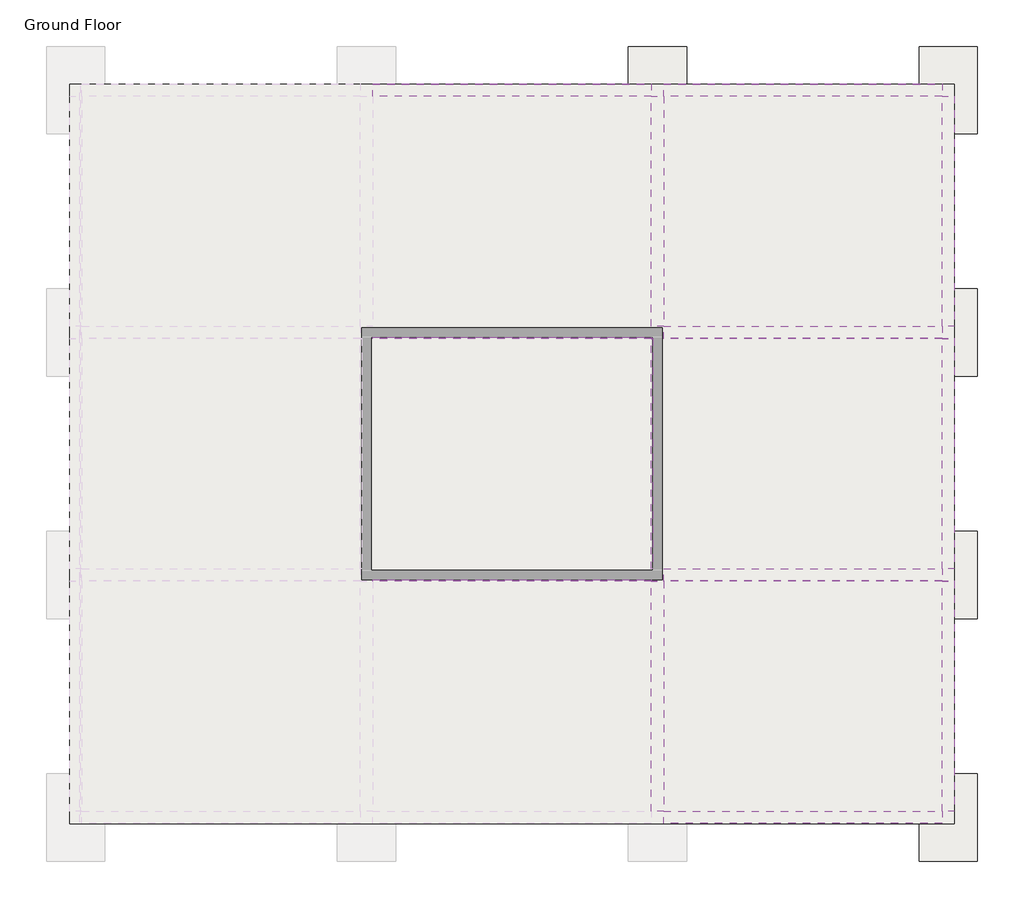
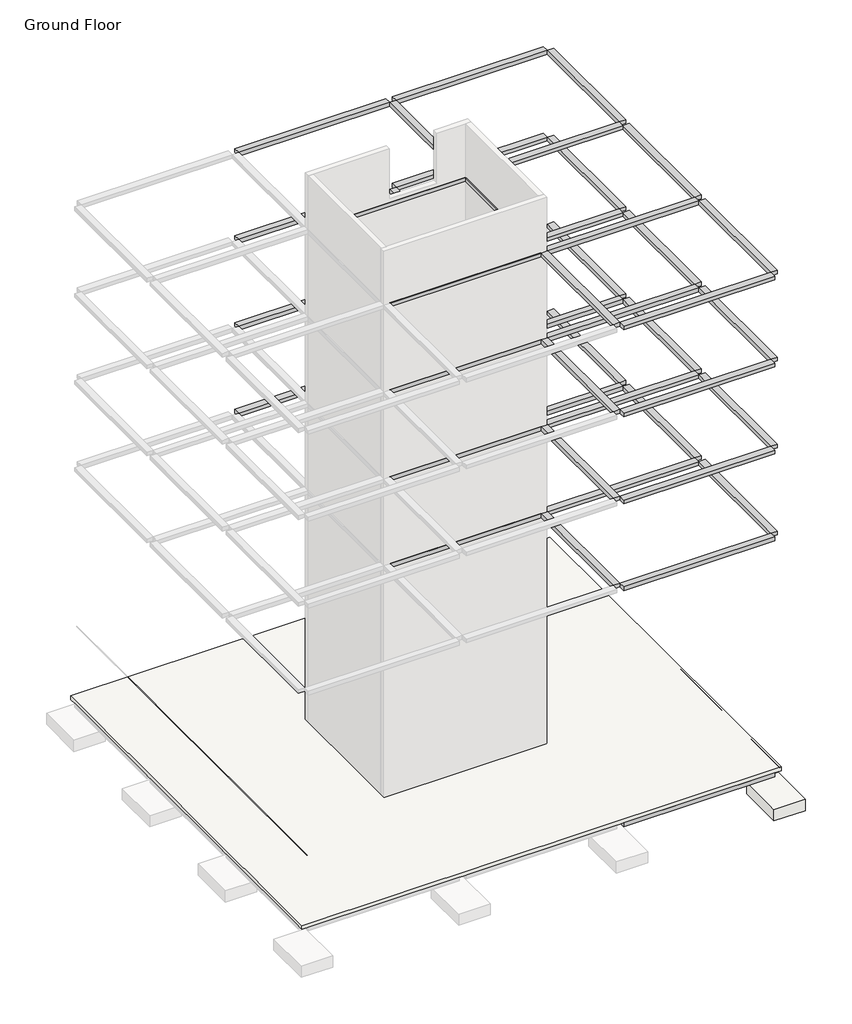
# One storey, part 2 of 3: 65 beams, 8 slabs.
"""IFC4 building model written with IfcOpenShell, lengths in millimetres."""

from ifc_helpers import new_model, si_unit, frame, origin, place, context, project, spatial, polyline, outline, extrude, faceted_brep, element, save

model = new_model("IFC4")

# Units and contexts
model_context = context("Model", 3, world=origin())
ifc_project = project(units=[si_unit("LENGTHUNIT", "METRE", prefix="MILLI")], contexts=[model_context])

# Site, building, storey
site = spatial("IfcSite", under=ifc_project)
building = spatial("IfcBuilding", under=site)
storey = spatial("IfcBuildingStorey", under=building, Name="Ground Floor", Elevation=2000.0)

# Beams
placement = place(None, origin())
element("IfcBeam", 1, ObjectType="Concrete-Rectangular Beam : 250 x 300mm", at=placement, inside=storey, context=model_context, shape_type="SweptSolid", body=[
    extrude(outline(polyline([(-2833.7181639, -5693.2383613), (-2833.7181639, -5443.2383613), (2916.2818361, -5443.2383613), (2916.2818361, -5693.2383613), (-2833.7181639, -5693.2383613)])), frame((0.0, 0.0, 1700.0), z_axis=(0.0, 0.0, 1.0), x_axis=(1.0, 0.0, 0.0)), (0.0, 0.0, 1.0), 150.0),
])
element("IfcBeam", 2, ObjectType="Concrete-Rectangular Beam : 250 x 300mm", at=placement, inside=storey, context=model_context, shape_type="SweptSolid", body=[
    extrude(outline(polyline([(3166.2818361, -5693.2383613), (3166.2818361, -5443.2383613), (8916.2818361, -5443.2383613), (8916.2818361, -5693.2383613), (3166.2818361, -5693.2383613)])), frame((0.0, 0.0, 1700.0), z_axis=(0.0, 0.0, 1.0), x_axis=(1.0, 0.0, 0.0)), (0.0, 0.0, 1.0), 150.0),
])
element("IfcBeam", 3, ObjectType="Concrete-Rectangular Beam : 250 x 300mm", at=placement, inside=storey, context=model_context, shape_type="SweptSolid", body=[
    extrude(outline(polyline([(3166.2818361, -10443.2383613), (2916.2818361, -10443.2383613), (2916.2818361, -5693.2383613), (3166.2818361, -5693.2383613), (3166.2818361, -10443.2383613)])), frame((0.0, 0.0, 1700.0), z_axis=(0.0, 0.0, 1.0), x_axis=(1.0, 0.0, 0.0)), (0.0, 0.0, 1.0), 150.0),
])
element("IfcBeam", 4, ObjectType="Concrete-Rectangular Beam : 250 x 300mm", at=placement, inside=storey, context=model_context, shape_type="SweptSolid", body=[
    extrude(outline(polyline([(2916.2818361, -15443.2383613), (2916.2818361, -10693.2383613), (2941.2818361, -10693.2383613), (2941.2818361, -15443.2383613), (2916.2818361, -15443.2383613)])), frame((0.0, 0.0, 1700.0), z_axis=(0.0, 0.0, 1.0), x_axis=(1.0, 0.0, 0.0)), (0.0, 0.0, 1.0), 150.0),
    extrude(outline(polyline([(3166.2818361, -10693.2383613), (3166.2818361, -15443.2383613), (3141.2818361, -15443.2383613), (3141.2818361, -10693.2383613), (3166.2818361, -10693.2383613)])), frame((0.0, 0.0, 1700.0), z_axis=(0.0, 0.0, 1.0), x_axis=(1.0, 0.0, 0.0)), (0.0, 0.0, 1.0), 150.0),
])
element("IfcBeam", 5, ObjectType="Concrete-Rectangular Beam : 250 x 300mm", at=placement, inside=storey, context=model_context, shape_type="SweptSolid", body=[
    extrude(outline(polyline([(3166.2818361, -20443.2383613), (2916.2818361, -20443.2383613), (2916.2818361, -15693.2383613), (3166.2818361, -15693.2383613), (3166.2818361, -20443.2383613)])), frame((0.0, 0.0, 1700.0), z_axis=(0.0, 0.0, 1.0), x_axis=(1.0, 0.0, 0.0)), (0.0, 0.0, 1.0), 150.0),
])
element("IfcBeam", 6, ObjectType="Concrete-Rectangular Beam : 250 x 300mm", at=placement, inside=storey, context=model_context, shape_type="SweptSolid", body=[
    extrude(outline(polyline([(9166.2818361, -10443.2383613), (8916.2818361, -10443.2383613), (8916.2818361, -5693.2383613), (9166.2818361, -5693.2383613), (9166.2818361, -10443.2383613)])), frame((0.0, 0.0, 1700.0), z_axis=(0.0, 0.0, 1.0), x_axis=(1.0, 0.0, 0.0)), (0.0, 0.0, 1.0), 150.0),
])
element("IfcBeam", 7, ObjectType="Concrete-Rectangular Beam : 250 x 300mm", at=placement, inside=storey, context=model_context, shape_type="SweptSolid", body=[
    extrude(outline(polyline([(9166.2818361, -15443.2383613), (8916.2818361, -15443.2383613), (8916.2818361, -10693.2383613), (9166.2818361, -10693.2383613), (9166.2818361, -15443.2383613)])), frame((0.0, 0.0, 1700.0), z_axis=(0.0, 0.0, 1.0), x_axis=(1.0, 0.0, 0.0)), (0.0, 0.0, 1.0), 150.0),
])
element("IfcBeam", 8, ObjectType="Concrete-Rectangular Beam : 250 x 300mm", at=placement, inside=storey, context=model_context, shape_type="SweptSolid", body=[
    extrude(outline(polyline([(9166.2818361, -20443.2383613), (8916.2818361, -20443.2383613), (8916.2818361, -15693.2383613), (9166.2818361, -15693.2383613), (9166.2818361, -20443.2383613)])), frame((0.0, 0.0, 1700.0), z_axis=(0.0, 0.0, 1.0), x_axis=(1.0, 0.0, 0.0)), (0.0, 0.0, 1.0), 150.0),
])
element("IfcBeam", 9, ObjectType="Concrete-Rectangular Beam : 250 x 300mm", at=placement, inside=storey, context=model_context, shape_type="SweptSolid", body=[
    extrude(outline(polyline([(3166.2818361, -20693.2383613), (3166.2818361, -20443.2383613), (8916.2818361, -20443.2383613), (8916.2818361, -20693.2383613), (3166.2818361, -20693.2383613)])), frame((0.0, 0.0, 1700.0), z_axis=(0.0, 0.0, 1.0), x_axis=(1.0, 0.0, 0.0)), (0.0, 0.0, 1.0), 150.0),
])
element("IfcBeam", 10, ObjectType="Concrete-Rectangular Beam : 250 x 300mm", at=placement, inside=storey, context=model_context, shape_type="SweptSolid", body=[
    extrude(outline(polyline([(2916.2818361, -15693.2383613), (-2833.7181639, -15693.2383613), (-2833.7181639, -15668.2383613), (2916.2818361, -15668.2383613), (2916.2818361, -15693.2383613)])), frame((0.0, 0.0, 1700.0), z_axis=(0.0, 0.0, 1.0), x_axis=(1.0, 0.0, 0.0)), (0.0, 0.0, 1.0), 150.0),
    extrude(outline(polyline([(-2833.7181639, -15443.2383613), (2916.2818361, -15443.2383613), (2916.2818361, -15468.2383613), (-2833.7181639, -15468.2383613), (-2833.7181639, -15443.2383613)])), frame((0.0, 0.0, 1700.0), z_axis=(0.0, 0.0, 1.0), x_axis=(1.0, 0.0, 0.0)), (0.0, 0.0, 1.0), 150.0),
])
element("IfcBeam", 11, ObjectType="Concrete-Rectangular Beam : 250 x 300mm", at=placement, inside=storey, context=model_context, shape_type="SweptSolid", body=[
    extrude(outline(polyline([(3166.2818361, -15693.2383613), (3166.2818361, -15443.2383613), (8916.2818361, -15443.2383613), (8916.2818361, -15693.2383613), (3166.2818361, -15693.2383613)])), frame((0.0, 0.0, 1700.0), z_axis=(0.0, 0.0, 1.0), x_axis=(1.0, 0.0, 0.0)), (0.0, 0.0, 1.0), 150.0),
])
element("IfcBeam", 12, ObjectType="Concrete-Rectangular Beam : 250 x 300mm", at=placement, inside=storey, context=model_context, shape_type="SweptSolid", body=[
    extrude(outline(polyline([(2916.2818361, -10693.2383613), (-2833.7181639, -10693.2383613), (-2833.7181639, -10668.2383613), (2916.2818361, -10668.2383613), (2916.2818361, -10693.2383613)])), frame((0.0, 0.0, 1700.0), z_axis=(0.0, 0.0, 1.0), x_axis=(1.0, 0.0, 0.0)), (0.0, 0.0, 1.0), 150.0),
    extrude(outline(polyline([(-2833.7181639, -10443.2383613), (2916.2818361, -10443.2383613), (2916.2818361, -10468.2383613), (-2833.7181639, -10468.2383613), (-2833.7181639, -10443.2383613)])), frame((0.0, 0.0, 1700.0), z_axis=(0.0, 0.0, 1.0), x_axis=(1.0, 0.0, 0.0)), (0.0, 0.0, 1.0), 150.0),
])
element("IfcBeam", 13, ObjectType="Concrete-Rectangular Beam : 250 x 300mm", at=placement, inside=storey, context=model_context, shape_type="SweptSolid", body=[
    extrude(outline(polyline([(3166.2818361, -10693.2383613), (3166.2818361, -10443.2383613), (8916.2818361, -10443.2383613), (8916.2818361, -10693.2383613), (3166.2818361, -10693.2383613)])), frame((0.0, 0.0, 1700.0), z_axis=(0.0, 0.0, 1.0), x_axis=(1.0, 0.0, 0.0)), (0.0, 0.0, 1.0), 150.0),
])
element("IfcBeam", 14, ObjectType="Concrete-Rectangular Beam : 250 x 300mm", at=placement, inside=storey, context=model_context, shape_type="SweptSolid", body=[
    extrude(outline(polyline([(-2833.7181639, -5693.2383613), (-2833.7181639, -5443.2383613), (2916.2818361, -5443.2383613), (2916.2818361, -5693.2383613), (-2833.7181639, -5693.2383613)])), frame((0.0, 0.0, 11200.0), z_axis=(0.0, 0.0, 1.0), x_axis=(1.0, 0.0, 0.0)), (0.0, 0.0, 1.0), 150.0),
])
element("IfcBeam", 15, ObjectType="Concrete-Rectangular Beam : 250 x 300mm", at=placement, inside=storey, context=model_context, shape_type="SweptSolid", body=[
    extrude(outline(polyline([(3166.2818361, -5693.2383613), (3166.2818361, -5443.2383613), (8916.2818361, -5443.2383613), (8916.2818361, -5693.2383613), (3166.2818361, -5693.2383613)])), frame((0.0, 0.0, 11200.0), z_axis=(0.0, 0.0, 1.0), x_axis=(1.0, 0.0, 0.0)), (0.0, 0.0, 1.0), 150.0),
])
element("IfcBeam", 16, ObjectType="Concrete-Rectangular Beam : 250 x 300mm", at=placement, inside=storey, context=model_context, shape_type="SweptSolid", body=[
    extrude(outline(polyline([(2916.2818361, -10443.2383613), (2916.2818361, -5693.2383613), (3166.2818361, -5693.2383613), (3166.2818361, -10443.2383613), (2916.2818361, -10443.2383613)])), frame((0.0, 0.0, 11200.0), z_axis=(0.0, 0.0, 1.0), x_axis=(1.0, 0.0, 0.0)), (0.0, 0.0, 1.0), 150.0),
])
element("IfcBeam", 17, ObjectType="Concrete-Rectangular Beam : 250 x 300mm", at=placement, inside=storey, context=model_context, shape_type="SweptSolid", body=[
    extrude(outline(polyline([(2916.2818361, -15443.2383613), (2916.2818361, -10693.2383613), (2941.2818361, -10693.2383613), (2941.2818361, -15443.2383613), (2916.2818361, -15443.2383613)])), frame((0.0, 0.0, 11200.0), z_axis=(0.0, 0.0, 1.0), x_axis=(1.0, 0.0, 0.0)), (0.0, 0.0, 1.0), 150.0),
    extrude(outline(polyline([(3166.2818361, -10693.2383613), (3166.2818361, -15443.2383613), (3141.2818361, -15443.2383613), (3141.2818361, -10693.2383613), (3166.2818361, -10693.2383613)])), frame((0.0, 0.0, 11200.0), z_axis=(0.0, 0.0, 1.0), x_axis=(1.0, 0.0, 0.0)), (0.0, 0.0, 1.0), 150.0),
])
element("IfcBeam", 18, ObjectType="Concrete-Rectangular Beam : 250 x 300mm", at=placement, inside=storey, context=model_context, shape_type="SweptSolid", body=[
    extrude(outline(polyline([(2916.2818361, -20443.2383613), (2916.2818361, -15693.2383613), (3166.2818361, -15693.2383613), (3166.2818361, -20443.2383613), (2916.2818361, -20443.2383613)])), frame((0.0, 0.0, 11200.0), z_axis=(0.0, 0.0, 1.0), x_axis=(1.0, 0.0, 0.0)), (0.0, 0.0, 1.0), 150.0),
])
element("IfcBeam", 19, ObjectType="Concrete-Rectangular Beam : 250 x 300mm", at=placement, inside=storey, context=model_context, shape_type="SweptSolid", body=[
    extrude(outline(polyline([(8916.2818361, -10443.2383613), (8916.2818361, -5693.2383613), (9166.2818361, -5693.2383613), (9166.2818361, -10443.2383613), (8916.2818361, -10443.2383613)])), frame((0.0, 0.0, 11200.0), z_axis=(0.0, 0.0, 1.0), x_axis=(1.0, 0.0, 0.0)), (0.0, 0.0, 1.0), 150.0),
])
element("IfcBeam", 20, ObjectType="Concrete-Rectangular Beam : 250 x 300mm", at=placement, inside=storey, context=model_context, shape_type="SweptSolid", body=[
    extrude(outline(polyline([(8916.2818361, -15443.2383613), (8916.2818361, -10693.2383613), (9166.2818361, -10693.2383613), (9166.2818361, -15443.2383613), (8916.2818361, -15443.2383613)])), frame((0.0, 0.0, 11200.0), z_axis=(0.0, 0.0, 1.0), x_axis=(1.0, 0.0, 0.0)), (0.0, 0.0, 1.0), 150.0),
])
element("IfcBeam", 21, ObjectType="Concrete-Rectangular Beam : 250 x 300mm", at=placement, inside=storey, context=model_context, shape_type="SweptSolid", body=[
    extrude(outline(polyline([(8916.2818361, -20443.2383613), (8916.2818361, -15693.2383613), (9166.2818361, -15693.2383613), (9166.2818361, -20443.2383613), (8916.2818361, -20443.2383613)])), frame((0.0, 0.0, 11200.0), z_axis=(0.0, 0.0, 1.0), x_axis=(1.0, 0.0, 0.0)), (0.0, 0.0, 1.0), 150.0),
])
element("IfcBeam", 22, ObjectType="Concrete-Rectangular Beam : 250 x 300mm", at=placement, inside=storey, context=model_context, shape_type="SweptSolid", body=[
    extrude(outline(polyline([(3166.2818361, -20443.2383613), (8916.2818361, -20443.2383613), (8916.2818361, -20693.2383613), (3166.2818361, -20693.2383613), (3166.2818361, -20443.2383613)])), frame((0.0, 0.0, 11200.0), z_axis=(0.0, 0.0, 1.0), x_axis=(1.0, 0.0, 0.0)), (0.0, 0.0, 1.0), 150.0),
])
element("IfcBeam", 23, ObjectType="Concrete-Rectangular Beam : 250 x 300mm", at=placement, inside=storey, context=model_context, shape_type="SweptSolid", body=[
    extrude(outline(polyline([(2916.2818361, -15693.2383613), (-2833.7181639, -15693.2383613), (-2833.7181639, -15668.2383613), (2916.2818361, -15668.2383613), (2916.2818361, -15693.2383613)])), frame((0.0, 0.0, 11200.0), z_axis=(0.0, 0.0, 1.0), x_axis=(1.0, 0.0, 0.0)), (0.0, 0.0, 1.0), 150.0),
    extrude(outline(polyline([(-2833.7181639, -15443.2383613), (2916.2818361, -15443.2383613), (2916.2818361, -15468.2383613), (-2833.7181639, -15468.2383613), (-2833.7181639, -15443.2383613)])), frame((0.0, 0.0, 11200.0), z_axis=(0.0, 0.0, 1.0), x_axis=(1.0, 0.0, 0.0)), (0.0, 0.0, 1.0), 150.0),
])
element("IfcBeam", 24, ObjectType="Concrete-Rectangular Beam : 250 x 300mm", at=placement, inside=storey, context=model_context, shape_type="SweptSolid", body=[
    extrude(outline(polyline([(3166.2818361, -15693.2383613), (3166.2818361, -15443.2383613), (8916.2818361, -15443.2383613), (8916.2818361, -15693.2383613), (3166.2818361, -15693.2383613)])), frame((0.0, 0.0, 11200.0), z_axis=(0.0, 0.0, 1.0), x_axis=(1.0, 0.0, 0.0)), (0.0, 0.0, 1.0), 150.0),
])
element("IfcBeam", 25, ObjectType="Concrete-Rectangular Beam : 250 x 300mm", at=placement, inside=storey, context=model_context, shape_type="SweptSolid", body=[
    extrude(outline(polyline([(2916.2818361, -10693.2383613), (-2833.7181639, -10693.2383613), (-2833.7181639, -10668.2383613), (2916.2818361, -10668.2383613), (2916.2818361, -10693.2383613)])), frame((0.0, 0.0, 11200.0), z_axis=(0.0, 0.0, 1.0), x_axis=(1.0, 0.0, 0.0)), (0.0, 0.0, 1.0), 150.0),
    extrude(outline(polyline([(-2833.7181639, -10443.2383613), (2916.2818361, -10443.2383613), (2916.2818361, -10468.2383613), (-2833.7181639, -10468.2383613), (-2833.7181639, -10443.2383613)])), frame((0.0, 0.0, 11200.0), z_axis=(0.0, 0.0, 1.0), x_axis=(1.0, 0.0, 0.0)), (0.0, 0.0, 1.0), 150.0),
])
element("IfcBeam", 26, ObjectType="Concrete-Rectangular Beam : 250 x 300mm", at=placement, inside=storey, context=model_context, shape_type="SweptSolid", body=[
    extrude(outline(polyline([(3166.2818361, -10693.2383613), (3166.2818361, -10443.2383613), (8916.2818361, -10443.2383613), (8916.2818361, -10693.2383613), (3166.2818361, -10693.2383613)])), frame((0.0, 0.0, 11200.0), z_axis=(0.0, 0.0, 1.0), x_axis=(1.0, 0.0, 0.0)), (0.0, 0.0, 1.0), 150.0),
])
element("IfcBeam", 27, ObjectType="Concrete-Rectangular Beam : 250 x 300mm", at=placement, inside=storey, context=model_context, shape_type="SweptSolid", body=[
    extrude(outline(polyline([(-2833.7181639, -5693.2383613), (-2833.7181639, -5443.2383613), (2916.2818361, -5443.2383613), (2916.2818361, -5693.2383613), (-2833.7181639, -5693.2383613)])), frame((0.0, 0.0, 14700.0), z_axis=(0.0, 0.0, 1.0), x_axis=(1.0, 0.0, 0.0)), (0.0, 0.0, 1.0), 150.0),
])
element("IfcBeam", 28, ObjectType="Concrete-Rectangular Beam : 250 x 300mm", at=placement, inside=storey, context=model_context, shape_type="SweptSolid", body=[
    extrude(outline(polyline([(3166.2818361, -5693.2383613), (3166.2818361, -5443.2383613), (8916.2818361, -5443.2383613), (8916.2818361, -5693.2383613), (3166.2818361, -5693.2383613)])), frame((0.0, 0.0, 14700.0), z_axis=(0.0, 0.0, 1.0), x_axis=(1.0, 0.0, 0.0)), (0.0, 0.0, 1.0), 150.0),
])
element("IfcBeam", 29, ObjectType="Concrete-Rectangular Beam : 250 x 300mm", at=placement, inside=storey, context=model_context, shape_type="SweptSolid", body=[
    extrude(outline(polyline([(2916.2818361, -10443.2383613), (2916.2818361, -5693.2383613), (3166.2818361, -5693.2383613), (3166.2818361, -10443.2383613), (2916.2818361, -10443.2383613)])), frame((0.0, 0.0, 14700.0), z_axis=(0.0, 0.0, 1.0), x_axis=(1.0, 0.0, 0.0)), (0.0, 0.0, 1.0), 150.0),
])
element("IfcBeam", 30, ObjectType="Concrete-Rectangular Beam : 250 x 300mm", at=placement, inside=storey, context=model_context, shape_type="SweptSolid", body=[
    extrude(outline(polyline([(2916.2818361, -15443.2383613), (2916.2818361, -10693.2383613), (2941.2818361, -10693.2383613), (2941.2818361, -15443.2383613), (2916.2818361, -15443.2383613)])), frame((0.0, 0.0, 14700.0), z_axis=(0.0, 0.0, 1.0), x_axis=(1.0, 0.0, 0.0)), (0.0, 0.0, 1.0), 150.0),
    extrude(outline(polyline([(3166.2818361, -10693.2383613), (3166.2818361, -15443.2383613), (3141.2818361, -15443.2383613), (3141.2818361, -10693.2383613), (3166.2818361, -10693.2383613)])), frame((0.0, 0.0, 14700.0), z_axis=(0.0, 0.0, 1.0), x_axis=(1.0, 0.0, 0.0)), (0.0, 0.0, 1.0), 150.0),
])
element("IfcBeam", 31, ObjectType="Concrete-Rectangular Beam : 250 x 300mm", at=placement, inside=storey, context=model_context, shape_type="SweptSolid", body=[
    extrude(outline(polyline([(2916.2818361, -20443.2383613), (2916.2818361, -15693.2383613), (3166.2818361, -15693.2383613), (3166.2818361, -20443.2383613), (2916.2818361, -20443.2383613)])), frame((0.0, 0.0, 14700.0), z_axis=(0.0, 0.0, 1.0), x_axis=(1.0, 0.0, 0.0)), (0.0, 0.0, 1.0), 150.0),
])
element("IfcBeam", 32, ObjectType="Concrete-Rectangular Beam : 250 x 300mm", at=placement, inside=storey, context=model_context, shape_type="SweptSolid", body=[
    extrude(outline(polyline([(8916.2818361, -10443.2383613), (8916.2818361, -5693.2383613), (9166.2818361, -5693.2383613), (9166.2818361, -10443.2383613), (8916.2818361, -10443.2383613)])), frame((0.0, 0.0, 14700.0), z_axis=(0.0, 0.0, 1.0), x_axis=(1.0, 0.0, 0.0)), (0.0, 0.0, 1.0), 150.0),
])
element("IfcBeam", 33, ObjectType="Concrete-Rectangular Beam : 250 x 300mm", at=placement, inside=storey, context=model_context, shape_type="SweptSolid", body=[
    extrude(outline(polyline([(8916.2818361, -15443.2383613), (8916.2818361, -10693.2383613), (9166.2818361, -10693.2383613), (9166.2818361, -15443.2383613), (8916.2818361, -15443.2383613)])), frame((0.0, 0.0, 14700.0), z_axis=(0.0, 0.0, 1.0), x_axis=(1.0, 0.0, 0.0)), (0.0, 0.0, 1.0), 150.0),
])
element("IfcBeam", 34, ObjectType="Concrete-Rectangular Beam : 250 x 300mm", at=placement, inside=storey, context=model_context, shape_type="SweptSolid", body=[
    extrude(outline(polyline([(8916.2818361, -20443.2383613), (8916.2818361, -15693.2383613), (9166.2818361, -15693.2383613), (9166.2818361, -20443.2383613), (8916.2818361, -20443.2383613)])), frame((0.0, 0.0, 14700.0), z_axis=(0.0, 0.0, 1.0), x_axis=(1.0, 0.0, 0.0)), (0.0, 0.0, 1.0), 150.0),
])
element("IfcBeam", 35, ObjectType="Concrete-Rectangular Beam : 250 x 300mm", at=placement, inside=storey, context=model_context, shape_type="SweptSolid", body=[
    extrude(outline(polyline([(3166.2818361, -20443.2383613), (8916.2818361, -20443.2383613), (8916.2818361, -20693.2383613), (3166.2818361, -20693.2383613), (3166.2818361, -20443.2383613)])), frame((0.0, 0.0, 14700.0), z_axis=(0.0, 0.0, 1.0), x_axis=(1.0, 0.0, 0.0)), (0.0, 0.0, 1.0), 150.0),
])
element("IfcBeam", 36, ObjectType="Concrete-Rectangular Beam : 250 x 300mm", at=placement, inside=storey, context=model_context, shape_type="SweptSolid", body=[
    extrude(outline(polyline([(2916.2818361, -15693.2383613), (-2833.7181639, -15693.2383613), (-2833.7181639, -15668.2383613), (2916.2818361, -15668.2383613), (2916.2818361, -15693.2383613)])), frame((0.0, 0.0, 14700.0), z_axis=(0.0, 0.0, 1.0), x_axis=(1.0, 0.0, 0.0)), (0.0, 0.0, 1.0), 150.0),
    extrude(outline(polyline([(-2833.7181639, -15443.2383613), (2916.2818361, -15443.2383613), (2916.2818361, -15468.2383613), (-2833.7181639, -15468.2383613), (-2833.7181639, -15443.2383613)])), frame((0.0, 0.0, 14700.0), z_axis=(0.0, 0.0, 1.0), x_axis=(1.0, 0.0, 0.0)), (0.0, 0.0, 1.0), 150.0),
])
element("IfcBeam", 37, ObjectType="Concrete-Rectangular Beam : 250 x 300mm", at=placement, inside=storey, context=model_context, shape_type="SweptSolid", body=[
    extrude(outline(polyline([(3166.2818361, -15693.2383613), (3166.2818361, -15443.2383613), (8916.2818361, -15443.2383613), (8916.2818361, -15693.2383613), (3166.2818361, -15693.2383613)])), frame((0.0, 0.0, 14700.0), z_axis=(0.0, 0.0, 1.0), x_axis=(1.0, 0.0, 0.0)), (0.0, 0.0, 1.0), 150.0),
])
element("IfcBeam", 38, ObjectType="Concrete-Rectangular Beam : 250 x 300mm", at=placement, inside=storey, context=model_context, shape_type="SweptSolid", body=[
    extrude(outline(polyline([(2916.2818361, -10693.2383613), (-2833.7181639, -10693.2383613), (-2833.7181639, -10668.2383613), (2916.2818361, -10668.2383613), (2916.2818361, -10693.2383613)])), frame((0.0, 0.0, 14700.0), z_axis=(0.0, 0.0, 1.0), x_axis=(1.0, 0.0, 0.0)), (0.0, 0.0, 1.0), 150.0),
    extrude(outline(polyline([(-2833.7181639, -10443.2383613), (2916.2818361, -10443.2383613), (2916.2818361, -10468.2383613), (-2833.7181639, -10468.2383613), (-2833.7181639, -10443.2383613)])), frame((0.0, 0.0, 14700.0), z_axis=(0.0, 0.0, 1.0), x_axis=(1.0, 0.0, 0.0)), (0.0, 0.0, 1.0), 150.0),
])
element("IfcBeam", 39, ObjectType="Concrete-Rectangular Beam : 250 x 300mm", at=placement, inside=storey, context=model_context, shape_type="SweptSolid", body=[
    extrude(outline(polyline([(3166.2818361, -10693.2383613), (3166.2818361, -10443.2383613), (8916.2818361, -10443.2383613), (8916.2818361, -10693.2383613), (3166.2818361, -10693.2383613)])), frame((0.0, 0.0, 14700.0), z_axis=(0.0, 0.0, 1.0), x_axis=(1.0, 0.0, 0.0)), (0.0, 0.0, 1.0), 150.0),
])
element("IfcBeam", 40, ObjectType="Concrete-Rectangular Beam : 250 x 300mm", at=placement, inside=storey, context=model_context, shape_type="SweptSolid", body=[
    extrude(outline(polyline([(-2833.7181639, -5693.2383613), (-2833.7181639, -5443.2383613), (2916.2818361, -5443.2383613), (2916.2818361, -5693.2383613), (-2833.7181639, -5693.2383613)])), frame((0.0, 0.0, 18200.0), z_axis=(0.0, 0.0, 1.0), x_axis=(1.0, 0.0, 0.0)), (0.0, 0.0, 1.0), 150.0),
])
element("IfcBeam", 41, ObjectType="Concrete-Rectangular Beam : 250 x 300mm", at=placement, inside=storey, context=model_context, shape_type="SweptSolid", body=[
    extrude(outline(polyline([(3166.2818361, -5693.2383613), (3166.2818361, -5443.2383613), (8916.2818361, -5443.2383613), (8916.2818361, -5693.2383613), (3166.2818361, -5693.2383613)])), frame((0.0, 0.0, 18200.0), z_axis=(0.0, 0.0, 1.0), x_axis=(1.0, 0.0, 0.0)), (0.0, 0.0, 1.0), 150.0),
])
element("IfcBeam", 42, ObjectType="Concrete-Rectangular Beam : 250 x 300mm", at=placement, inside=storey, context=model_context, shape_type="SweptSolid", body=[
    extrude(outline(polyline([(2916.2818361, -10443.2383613), (2916.2818361, -5693.2383613), (3166.2818361, -5693.2383613), (3166.2818361, -10443.2383613), (2916.2818361, -10443.2383613)])), frame((0.0, 0.0, 18200.0), z_axis=(0.0, 0.0, 1.0), x_axis=(1.0, 0.0, 0.0)), (0.0, 0.0, 1.0), 150.0),
])
element("IfcBeam", 43, ObjectType="Concrete-Rectangular Beam : 250 x 300mm", at=placement, inside=storey, context=model_context, shape_type="SweptSolid", body=[
    extrude(outline(polyline([(2916.2818361, -15443.2383613), (2916.2818361, -10693.2383613), (2941.2818361, -10693.2383613), (2941.2818361, -15443.2383613), (2916.2818361, -15443.2383613)])), frame((0.0, 0.0, 18200.0), z_axis=(0.0, 0.0, 1.0), x_axis=(1.0, 0.0, 0.0)), (0.0, 0.0, 1.0), 150.0),
    extrude(outline(polyline([(3166.2818361, -10693.2383613), (3166.2818361, -15443.2383613), (3141.2818361, -15443.2383613), (3141.2818361, -10693.2383613), (3166.2818361, -10693.2383613)])), frame((0.0, 0.0, 18200.0), z_axis=(0.0, 0.0, 1.0), x_axis=(1.0, 0.0, 0.0)), (0.0, 0.0, 1.0), 150.0),
])
element("IfcBeam", 44, ObjectType="Concrete-Rectangular Beam : 250 x 300mm", at=placement, inside=storey, context=model_context, shape_type="SweptSolid", body=[
    extrude(outline(polyline([(2916.2818361, -20443.2383613), (2916.2818361, -15693.2383613), (3166.2818361, -15693.2383613), (3166.2818361, -20443.2383613), (2916.2818361, -20443.2383613)])), frame((0.0, 0.0, 18200.0), z_axis=(0.0, 0.0, 1.0), x_axis=(1.0, 0.0, 0.0)), (0.0, 0.0, 1.0), 150.0),
])
element("IfcBeam", 45, ObjectType="Concrete-Rectangular Beam : 250 x 300mm", at=placement, inside=storey, context=model_context, shape_type="SweptSolid", body=[
    extrude(outline(polyline([(8916.2818361, -10443.2383613), (8916.2818361, -5693.2383613), (9166.2818361, -5693.2383613), (9166.2818361, -10443.2383613), (8916.2818361, -10443.2383613)])), frame((0.0, 0.0, 18200.0), z_axis=(0.0, 0.0, 1.0), x_axis=(1.0, 0.0, 0.0)), (0.0, 0.0, 1.0), 150.0),
])
element("IfcBeam", 46, ObjectType="Concrete-Rectangular Beam : 250 x 300mm", at=placement, inside=storey, context=model_context, shape_type="SweptSolid", body=[
    extrude(outline(polyline([(8916.2818361, -15443.2383613), (8916.2818361, -10693.2383613), (9166.2818361, -10693.2383613), (9166.2818361, -15443.2383613), (8916.2818361, -15443.2383613)])), frame((0.0, 0.0, 18200.0), z_axis=(0.0, 0.0, 1.0), x_axis=(1.0, 0.0, 0.0)), (0.0, 0.0, 1.0), 150.0),
])
element("IfcBeam", 47, ObjectType="Concrete-Rectangular Beam : 250 x 300mm", at=placement, inside=storey, context=model_context, shape_type="SweptSolid", body=[
    extrude(outline(polyline([(8916.2818361, -20443.2383613), (8916.2818361, -15693.2383613), (9166.2818361, -15693.2383613), (9166.2818361, -20443.2383613), (8916.2818361, -20443.2383613)])), frame((0.0, 0.0, 18200.0), z_axis=(0.0, 0.0, 1.0), x_axis=(1.0, 0.0, 0.0)), (0.0, 0.0, 1.0), 150.0),
])
element("IfcBeam", 48, ObjectType="Concrete-Rectangular Beam : 250 x 300mm", at=placement, inside=storey, context=model_context, shape_type="SweptSolid", body=[
    extrude(outline(polyline([(3166.2818361, -20443.2383613), (8916.2818361, -20443.2383613), (8916.2818361, -20693.2383613), (3166.2818361, -20693.2383613), (3166.2818361, -20443.2383613)])), frame((0.0, 0.0, 18200.0), z_axis=(0.0, 0.0, 1.0), x_axis=(1.0, 0.0, 0.0)), (0.0, 0.0, 1.0), 150.0),
])
element("IfcBeam", 49, ObjectType="Concrete-Rectangular Beam : 250 x 300mm", at=placement, inside=storey, context=model_context, shape_type="SweptSolid", body=[
    extrude(outline(polyline([(2916.2818361, -15693.2383613), (-2833.7181639, -15693.2383613), (-2833.7181639, -15668.2383613), (2916.2818361, -15668.2383613), (2916.2818361, -15693.2383613)])), frame((0.0, 0.0, 18200.0), z_axis=(0.0, 0.0, 1.0), x_axis=(1.0, 0.0, 0.0)), (0.0, 0.0, 1.0), 150.0),
    extrude(outline(polyline([(-2833.7181639, -15443.2383613), (2916.2818361, -15443.2383613), (2916.2818361, -15468.2383613), (-2833.7181639, -15468.2383613), (-2833.7181639, -15443.2383613)])), frame((0.0, 0.0, 18200.0), z_axis=(0.0, 0.0, 1.0), x_axis=(1.0, 0.0, 0.0)), (0.0, 0.0, 1.0), 150.0),
])
element("IfcBeam", 50, ObjectType="Concrete-Rectangular Beam : 250 x 300mm", at=placement, inside=storey, context=model_context, shape_type="SweptSolid", body=[
    extrude(outline(polyline([(3166.2818361, -15693.2383613), (3166.2818361, -15443.2383613), (8916.2818361, -15443.2383613), (8916.2818361, -15693.2383613), (3166.2818361, -15693.2383613)])), frame((0.0, 0.0, 18200.0), z_axis=(0.0, 0.0, 1.0), x_axis=(1.0, 0.0, 0.0)), (0.0, 0.0, 1.0), 150.0),
])
element("IfcBeam", 51, ObjectType="Concrete-Rectangular Beam : 250 x 300mm", at=placement, inside=storey, context=model_context, shape_type="SweptSolid", body=[
    extrude(outline(polyline([(2916.2818361, -10693.2383613), (-2833.7181639, -10693.2383613), (-2833.7181639, -10668.2383613), (2916.2818361, -10668.2383613), (2916.2818361, -10693.2383613)])), frame((0.0, 0.0, 18200.0), z_axis=(0.0, 0.0, 1.0), x_axis=(1.0, 0.0, 0.0)), (0.0, 0.0, 1.0), 150.0),
    extrude(outline(polyline([(-2833.7181639, -10443.2383613), (2916.2818361, -10443.2383613), (2916.2818361, -10468.2383613), (-2833.7181639, -10468.2383613), (-2833.7181639, -10443.2383613)])), frame((0.0, 0.0, 18200.0), z_axis=(0.0, 0.0, 1.0), x_axis=(1.0, 0.0, 0.0)), (0.0, 0.0, 1.0), 150.0),
])
element("IfcBeam", 52, ObjectType="Concrete-Rectangular Beam : 250 x 300mm", at=placement, inside=storey, context=model_context, shape_type="SweptSolid", body=[
    extrude(outline(polyline([(3166.2818361, -10693.2383613), (3166.2818361, -10443.2383613), (8916.2818361, -10443.2383613), (8916.2818361, -10693.2383613), (3166.2818361, -10693.2383613)])), frame((0.0, 0.0, 18200.0), z_axis=(0.0, 0.0, 1.0), x_axis=(1.0, 0.0, 0.0)), (0.0, 0.0, 1.0), 150.0),
])
element("IfcBeam", 53, ObjectType="Concrete-Rectangular Beam : 250 x 300mm", at=placement, inside=storey, context=model_context, shape_type="SweptSolid", body=[
    extrude(outline(polyline([(-2833.7181639, -5693.2383613), (-2833.7181639, -5443.2383613), (2916.2818361, -5443.2383613), (2916.2818361, -5693.2383613), (-2833.7181639, -5693.2383613)])), frame((0.0, 0.0, 21700.0), z_axis=(0.0, 0.0, 1.0), x_axis=(1.0, 0.0, 0.0)), (0.0, 0.0, 1.0), 150.0),
])
element("IfcBeam", 54, ObjectType="Concrete-Rectangular Beam : 250 x 300mm", at=placement, inside=storey, context=model_context, shape_type="SweptSolid", body=[
    extrude(outline(polyline([(3166.2818361, -5693.2383613), (3166.2818361, -5443.2383613), (8916.2818361, -5443.2383613), (8916.2818361, -5693.2383613), (3166.2818361, -5693.2383613)])), frame((0.0, 0.0, 21700.0), z_axis=(0.0, 0.0, 1.0), x_axis=(1.0, 0.0, 0.0)), (0.0, 0.0, 1.0), 150.0),
])
element("IfcBeam", 55, ObjectType="Concrete-Rectangular Beam : 250 x 300mm", at=placement, inside=storey, context=model_context, shape_type="SweptSolid", body=[
    extrude(outline(polyline([(2916.2818361, -10443.2383613), (2916.2818361, -5693.2383613), (3166.2818361, -5693.2383613), (3166.2818361, -10443.2383613), (2916.2818361, -10443.2383613)])), frame((0.0, 0.0, 21700.0), z_axis=(0.0, 0.0, 1.0), x_axis=(1.0, 0.0, 0.0)), (0.0, 0.0, 1.0), 150.0),
])
element("IfcBeam", 56, ObjectType="Concrete-Rectangular Beam : 250 x 300mm", at=placement, inside=storey, context=model_context, shape_type="SweptSolid", body=[
    extrude(outline(polyline([(2916.2818361, -15443.2383613), (2916.2818361, -10693.2383613), (2941.2818361, -10693.2383613), (2941.2818361, -15443.2383613), (2916.2818361, -15443.2383613)])), frame((0.0, 0.0, 21700.0), z_axis=(0.0, 0.0, 1.0), x_axis=(1.0, 0.0, 0.0)), (0.0, 0.0, 1.0), 150.0),
    extrude(outline(polyline([(3166.2818361, -10693.2383613), (3166.2818361, -15443.2383613), (3141.2818361, -15443.2383613), (3141.2818361, -10693.2383613), (3166.2818361, -10693.2383613)])), frame((0.0, 0.0, 21700.0), z_axis=(0.0, 0.0, 1.0), x_axis=(1.0, 0.0, 0.0)), (0.0, 0.0, 1.0), 150.0),
])
element("IfcBeam", 57, ObjectType="Concrete-Rectangular Beam : 250 x 300mm", at=placement, inside=storey, context=model_context, shape_type="SweptSolid", body=[
    extrude(outline(polyline([(2916.2818361, -20443.2383613), (2916.2818361, -15693.2383613), (3166.2818361, -15693.2383613), (3166.2818361, -20443.2383613), (2916.2818361, -20443.2383613)])), frame((0.0, 0.0, 21700.0), z_axis=(0.0, 0.0, 1.0), x_axis=(1.0, 0.0, 0.0)), (0.0, 0.0, 1.0), 150.0),
])
element("IfcBeam", 58, ObjectType="Concrete-Rectangular Beam : 250 x 300mm", at=placement, inside=storey, context=model_context, shape_type="SweptSolid", body=[
    extrude(outline(polyline([(8916.2818361, -10443.2383613), (8916.2818361, -5693.2383613), (9166.2818361, -5693.2383613), (9166.2818361, -10443.2383613), (8916.2818361, -10443.2383613)])), frame((0.0, 0.0, 21700.0), z_axis=(0.0, 0.0, 1.0), x_axis=(1.0, 0.0, 0.0)), (0.0, 0.0, 1.0), 150.0),
])
element("IfcBeam", 59, ObjectType="Concrete-Rectangular Beam : 250 x 300mm", at=placement, inside=storey, context=model_context, shape_type="SweptSolid", body=[
    extrude(outline(polyline([(8916.2818361, -15443.2383613), (8916.2818361, -10693.2383613), (9166.2818361, -10693.2383613), (9166.2818361, -15443.2383613), (8916.2818361, -15443.2383613)])), frame((0.0, 0.0, 21700.0), z_axis=(0.0, 0.0, 1.0), x_axis=(1.0, 0.0, 0.0)), (0.0, 0.0, 1.0), 150.0),
])
element("IfcBeam", 60, ObjectType="Concrete-Rectangular Beam : 250 x 300mm", at=placement, inside=storey, context=model_context, shape_type="SweptSolid", body=[
    extrude(outline(polyline([(8916.2818361, -20443.2383613), (8916.2818361, -15693.2383613), (9166.2818361, -15693.2383613), (9166.2818361, -20443.2383613), (8916.2818361, -20443.2383613)])), frame((0.0, 0.0, 21700.0), z_axis=(0.0, 0.0, 1.0), x_axis=(1.0, 0.0, 0.0)), (0.0, 0.0, 1.0), 150.0),
])
element("IfcBeam", 61, ObjectType="Concrete-Rectangular Beam : 250 x 300mm", at=placement, inside=storey, context=model_context, shape_type="SweptSolid", body=[
    extrude(outline(polyline([(3166.2818361, -20443.2383613), (8916.2818361, -20443.2383613), (8916.2818361, -20693.2383613), (3166.2818361, -20693.2383613), (3166.2818361, -20443.2383613)])), frame((0.0, 0.0, 21700.0), z_axis=(0.0, 0.0, 1.0), x_axis=(1.0, 0.0, 0.0)), (0.0, 0.0, 1.0), 150.0),
])
element("IfcBeam", 62, ObjectType="Concrete-Rectangular Beam : 250 x 300mm", at=placement, inside=storey, context=model_context, shape_type="SweptSolid", body=[
    extrude(outline(polyline([(2916.2818361, -15693.2383613), (-2833.7181639, -15693.2383613), (-2833.7181639, -15668.2383613), (2916.2818361, -15668.2383613), (2916.2818361, -15693.2383613)])), frame((0.0, 0.0, 21700.0), z_axis=(0.0, 0.0, 1.0), x_axis=(1.0, 0.0, 0.0)), (0.0, 0.0, 1.0), 150.0),
    extrude(outline(polyline([(-2833.7181639, -15443.2383613), (2916.2818361, -15443.2383613), (2916.2818361, -15468.2383613), (-2833.7181639, -15468.2383613), (-2833.7181639, -15443.2383613)])), frame((0.0, 0.0, 21700.0), z_axis=(0.0, 0.0, 1.0), x_axis=(1.0, 0.0, 0.0)), (0.0, 0.0, 1.0), 150.0),
])
element("IfcBeam", 63, ObjectType="Concrete-Rectangular Beam : 250 x 300mm", at=placement, inside=storey, context=model_context, shape_type="SweptSolid", body=[
    extrude(outline(polyline([(3166.2818361, -15693.2383613), (3166.2818361, -15443.2383613), (8916.2818361, -15443.2383613), (8916.2818361, -15693.2383613), (3166.2818361, -15693.2383613)])), frame((0.0, 0.0, 21700.0), z_axis=(0.0, 0.0, 1.0), x_axis=(1.0, 0.0, 0.0)), (0.0, 0.0, 1.0), 150.0),
])
element("IfcBeam", 64, ObjectType="Concrete-Rectangular Beam : 250 x 300mm", at=placement, inside=storey, context=model_context, shape_type="SweptSolid", body=[
    extrude(outline(polyline([(2916.2818361, -10693.2383613), (-2833.7181639, -10693.2383613), (-2833.7181639, -10668.2383613), (2916.2818361, -10668.2383613), (2916.2818361, -10693.2383613)])), frame((0.0, 0.0, 21700.0), z_axis=(0.0, 0.0, 1.0), x_axis=(1.0, 0.0, 0.0)), (0.0, 0.0, 1.0), 150.0),
    extrude(outline(polyline([(-2833.7181639, -10443.2383613), (2916.2818361, -10443.2383613), (2916.2818361, -10468.2383613), (-2833.7181639, -10468.2383613), (-2833.7181639, -10443.2383613)])), frame((0.0, 0.0, 21700.0), z_axis=(0.0, 0.0, 1.0), x_axis=(1.0, 0.0, 0.0)), (0.0, 0.0, 1.0), 150.0),
])
element("IfcBeam", 65, ObjectType="Concrete-Rectangular Beam : 250 x 300mm", at=placement, inside=storey, context=model_context, shape_type="SweptSolid", body=[
    extrude(outline(polyline([(3166.2818361, -10443.2383613), (8916.2818361, -10443.2383613), (8916.2818361, -10693.2383613), (3166.2818361, -10693.2383613), (3166.2818361, -10443.2383613)])), frame((0.0, 0.0, 21700.0), z_axis=(0.0, 0.0, 1.0), x_axis=(1.0, 0.0, 0.0)), (0.0, 0.0, 1.0), 150.0),
])

# Slabs
element("IfcSlab", 66, ObjectType="150mm Foundation Slab", at=placement, inside=storey, context=model_context, shape_type="Brep", body=[
    faceted_brep([(-9083.7181639, -5443.2383613, 1850.0), (-8833.7181639, -5443.2383613, 1850.0), (-3083.7181639, -5443.2383613, 1850.0), (-2833.7181639, -5443.2383613, 1850.0), (2916.2818361, -5443.2383613, 1850.0), (3166.2818361, -5443.2383613, 1850.0), (8916.2818361, -5443.2383613, 1850.0), (9166.2818361, -5443.2383613, 1850.0), (9166.2818361, -5693.2383613, 1850.0), (9166.2818361, -10443.2383613, 1850.0), (9166.2818361, -10693.2383613, 1850.0), (9166.2818361, -15443.2383613, 1850.0), (9166.2818361, -15693.2383613, 1850.0), (9166.2818361, -20443.2383613, 1850.0), (9166.2818361, -20693.2383613, 1850.0), (8916.2818361, -20693.2383613, 1850.0), (3166.2818361, -20693.2383613, 1850.0), (2916.2818361, -20693.2383613, 1850.0), (-2833.7181639, -20693.2383613, 1850.0), (-3083.7181639, -20693.2383613, 1850.0), (-8833.7181639, -20693.2383613, 1850.0), (-9083.7181639, -20693.2383613, 1850.0), (-9083.7181639, -20443.2383613, 1850.0), (-9083.7181639, -15693.2383613, 1850.0), (-9083.7181639, -15443.2383613, 1850.0), (-9083.7181639, -10693.2383613, 1850.0), (-9083.7181639, -10443.2383613, 1850.0), (-9083.7181639, -5693.2383613, 1850.0), (-9083.7181639, -5443.2383613, 2000.0), (-9083.7181639, -20693.2383613, 2000.0), (9166.2818361, -20693.2383613, 2000.0), (9166.2818361, -5443.2383613, 2000.0)], [[[0, 1, 2, 3, 4, 5, 6, 7, 8, 9, 10, 11, 12, 13, 14, 15, 16, 17, 18, 19, 20, 21, 22, 23, 24, 25, 26, 27]], [[28, 29, 30, 31]], [[7, 6, 5, 4, 3, 2, 1, 0, 28, 31]], [[14, 13, 12, 11, 10, 9, 8, 7, 31, 30]], [[21, 20, 19, 18, 17, 16, 15, 14, 30, 29]], [[0, 27, 26, 25, 24, 23, 22, 21, 29, 28]]]),
])
element("IfcSlab", 67, ObjectType="Footing-Rectangular : 1800 x 1200 x 450mm", at=placement, inside=storey, context=model_context, shape_type="SweptSolid", body=[
    extrude(outline(polyline([(3641.2818361, -14668.2383613), (3641.2818361, -16468.2383613), (2441.2818361, -16468.2383613), (2441.2818361, -14668.2383613), (3641.2818361, -14668.2383613)])), frame((0.0, 0.0, 550.0), z_axis=(0.0, 0.0, 1.0), x_axis=(1.0, 0.0, 0.0)), (0.0, 0.0, 1.0), 450.0),
])
element("IfcSlab", 68, ObjectType="Footing-Rectangular : 1800 x 1200 x 450mm", at=placement, inside=storey, context=model_context, shape_type="SweptSolid", body=[
    extrude(outline(polyline([(3641.2818361, -9668.2383613), (3641.2818361, -11468.2383613), (2441.2818361, -11468.2383613), (2441.2818361, -9668.2383613), (3641.2818361, -9668.2383613)])), frame((0.0, 0.0, 550.0), z_axis=(0.0, 0.0, 1.0), x_axis=(1.0, 0.0, 0.0)), (0.0, 0.0, 1.0), 450.0),
])
element("IfcSlab", 69, ObjectType="Footing-Rectangular : 1800 x 1200 x 450mm", at=placement, inside=storey, context=model_context, shape_type="SweptSolid", body=[
    extrude(outline(polyline([(3641.2818361, -4668.2383613), (3641.2818361, -6468.2383613), (2441.2818361, -6468.2383613), (2441.2818361, -4668.2383613), (3641.2818361, -4668.2383613)])), frame((0.0, 0.0, 550.0), z_axis=(0.0, 0.0, 1.0), x_axis=(1.0, 0.0, 0.0)), (0.0, 0.0, 1.0), 450.0),
])
element("IfcSlab", 70, ObjectType="Footing-Rectangular : 1800 x 1200 x 450mm", at=placement, inside=storey, context=model_context, shape_type="SweptSolid", body=[
    extrude(outline(polyline([(9641.2818361, -19668.2383613), (9641.2818361, -21468.2383613), (8441.2818361, -21468.2383613), (8441.2818361, -19668.2383613), (9641.2818361, -19668.2383613)])), frame((0.0, 0.0, 550.0), z_axis=(0.0, 0.0, 1.0), x_axis=(1.0, 0.0, 0.0)), (0.0, 0.0, 1.0), 450.0),
])
element("IfcSlab", 71, ObjectType="Footing-Rectangular : 1800 x 1200 x 450mm", at=placement, inside=storey, context=model_context, shape_type="SweptSolid", body=[
    extrude(outline(polyline([(9641.2818361, -14668.2383613), (9641.2818361, -16468.2383613), (8441.2818361, -16468.2383613), (8441.2818361, -14668.2383613), (9641.2818361, -14668.2383613)])), frame((0.0, 0.0, 550.0), z_axis=(0.0, 0.0, 1.0), x_axis=(1.0, 0.0, 0.0)), (0.0, 0.0, 1.0), 450.0),
])
element("IfcSlab", 72, ObjectType="Footing-Rectangular : 1800 x 1200 x 450mm", at=placement, inside=storey, context=model_context, shape_type="SweptSolid", body=[
    extrude(outline(polyline([(9641.2818361, -9668.2383613), (9641.2818361, -11468.2383613), (8441.2818361, -11468.2383613), (8441.2818361, -9668.2383613), (9641.2818361, -9668.2383613)])), frame((0.0, 0.0, 550.0), z_axis=(0.0, 0.0, 1.0), x_axis=(1.0, 0.0, 0.0)), (0.0, 0.0, 1.0), 450.0),
])
element("IfcSlab", 73, ObjectType="Footing-Rectangular : 1800 x 1200 x 450mm", at=placement, inside=storey, context=model_context, shape_type="SweptSolid", body=[
    extrude(outline(polyline([(8441.2818361, -6468.2383613), (8441.2818361, -4668.2383613), (9641.2818361, -4668.2383613), (9641.2818361, -6468.2383613), (8441.2818361, -6468.2383613)])), frame((0.0, 0.0, 550.0), z_axis=(0.0, 0.0, 1.0), x_axis=(1.0, 0.0, 0.0)), (0.0, 0.0, 1.0), 450.0),
])

save(model, "model.ifc")

# Revit data of these elements
# Type "Concrete-Rectangular Beam : 250 x 300mm"
#   Length [instance default] = 1524 mm
#   b = 250 mm
#   h = 300 mm
#   Structural Material [instance default] = Concrete, Cast-in-Place gray
#   Assembly Code = ""
# Type "150mm Foundation Slab"
#   Layers, outside or top first: 150 mm "Concrete, Cast-in-Place gray" (function 1)
# Type "Footing-Rectangular : 1800 x 1200 x 450mm"
#   Width = 1200 mm
#   Length = 1800 mm
#   Foundation Thickness = 450 mm
#   Structural Material [instance default] = Concrete - Cast-in-Place Concrete
#   Assembly Code = ""
# Elements 1, 2, 3, 4, 5, 6, 7, 8, 9, 10, 11, 12, 13, 14, 15, 16, 17, 18, 19, 20, 21, 22, 23, 24, 25, 26, 27, 28, 29, 30, 31, 32, 33, 34, 35, 36, 37, 38, 39, 40, 41, 42, 43, 44, 45, 46, 47, 48, 49, 50, 51, 52, 53, 54, 55, 56, 57, 58, 59, 60, 61, 62, 63, 64, 65 (IfcBeam, "Concrete-Rectangular Beam : 250 x 300mm")
#   Structural Material = Concrete, Cast-in-Place gray
#   Phase Created = New Construction
#   Materials on its faces: "Concrete, Cast-in-Place gray"
# Element 66 (IfcSlab, "150mm Foundation Slab")
#   built-in parameter 1001955 = 3.14159 (stored number, unit not read)
#   Height Offset From Level = 0 mm
#   built-in parameter 1001954 = 1
#   Phase Created = New Construction
#   Materials on its faces: "Concrete, Cast-in-Place gray"
# Elements 67, 68, 69, 70, 71, 72, 73 (IfcSlab, "Footing-Rectangular : 1800 x 1200 x 450mm")
#   Structural Material = Concrete - Cast-in-Place Concrete
#   Phase Created = New Construction
#   Materials on its faces: "Concrete - Cast-in-Place Concrete"
# Materials
#   "Concrete, Cast-in-Place gray": class "Concrete", colour RGB 192 192 192, transparency 0, Description = "Cast-in-place concrete", Cost = 0
#   "Concrete - Cast-in-Place Concrete": class "Concrete", colour RGB 192 192 192, transparency 0, Cost = 0
